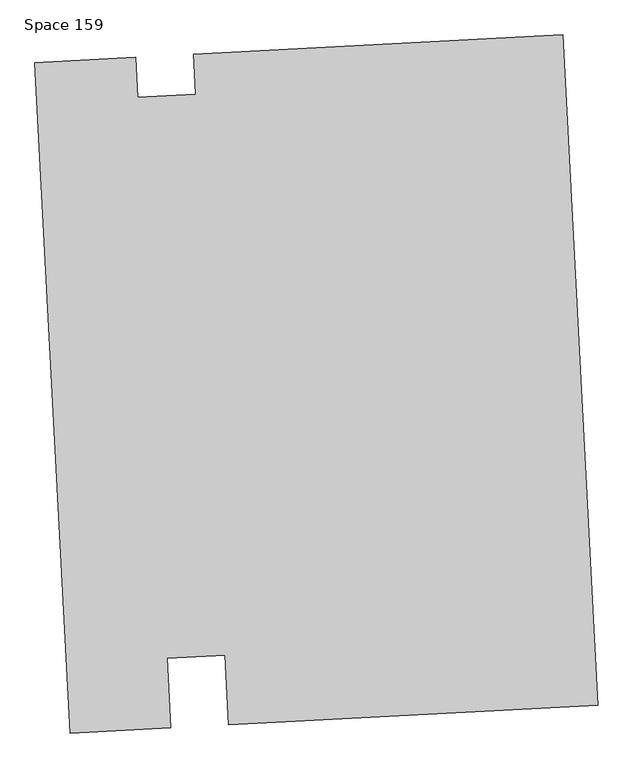
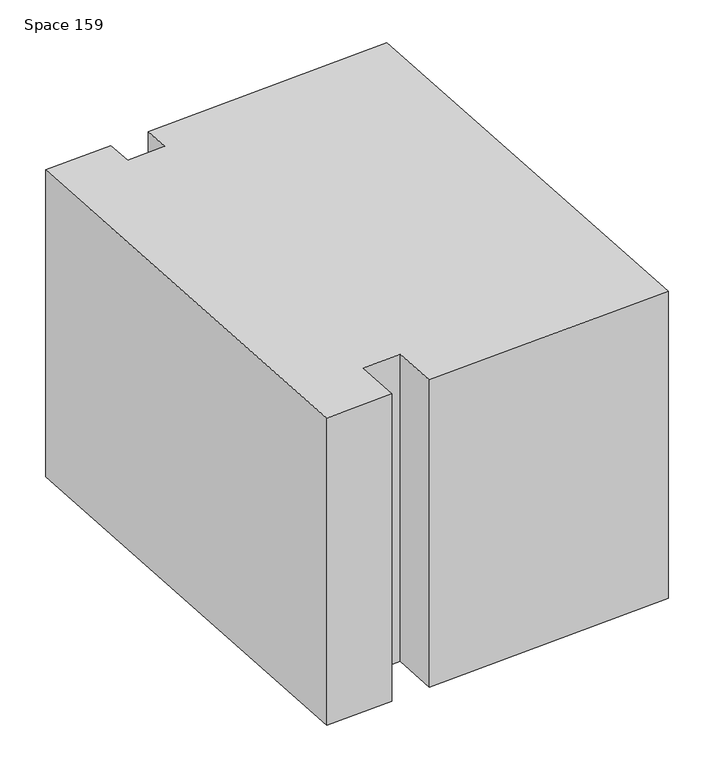
"""IFC4 building model written with IfcOpenShell, lengths in millimetres: proxy geometry, Space 159."""

from ifc_helpers import new_model, si_unit, frame, origin, place, context, project, spatial, polyline, outline, extrude, source, transform, mapped, element, save


def space_159_557c9301(model_context):
    return source(origin(), model_context, "Body", "SweptSolid", [
        extrude(outline(polyline([(-1342.871722, -35427.1773851), (-1365.6365546, -34992.7985032), (-1727.0905147, -35011.7415026), (-1704.3256821, -35446.1203845), (-2335.2847879, -35479.18755), (-2554.9571138, -31287.5898723), (-1923.998008, -31254.5227068), (-1910.8708418, -31505.0039598), (-1549.4168817, -31486.0609604), (-1562.5440479, -31235.5797074), (748.8589075, -31114.4442115), (968.5312334, -35306.0418892), (-1342.871722, -35427.1773851)])), frame((0.0, 0.0, 3810.0), z_axis=(0.0, 0.0, 1.0), x_axis=(1.0, 0.0, 0.0)), (0.0, 0.0, 1.0), 3048.0),
    ])


if __name__ == "__main__":
    model = new_model("IFC4")
    model_context = context("Model", 3, world=origin())
    ifc_project = project(units=[si_unit("LENGTHUNIT", "METRE", prefix="MILLI")], contexts=[model_context])
    site = spatial("IfcSite", under=ifc_project)
    building = spatial("IfcBuilding", under=site)
    placement = place(None, origin())
    space_159_shape = space_159_557c9301(model_context)
    element("IfcBuildingElementProxy", 1, Name="Space 159", ObjectType="Space 159", at=placement, inside=building, context=model_context, shape_type="MappedRepresentation", body=[
        mapped(space_159_shape, transform((0.0, 0.0, 0.0), x_axis=(1.0, 0.0, 0.0), y_axis=(0.0, 1.0, 0.0), z_axis=(0.0, 0.0, 1.0))),
    ])
    save(model, "model.ifc")

# Revit data of these elements
# Element 1 (IfcBuildingElementProxy, "Space 159")
#   Materials on its faces: "Render Material 255-255-255"
# Materials
#   "Render Material 255-255-255": class "Unassigned", colour RGB 255 255 255, transparency 0
